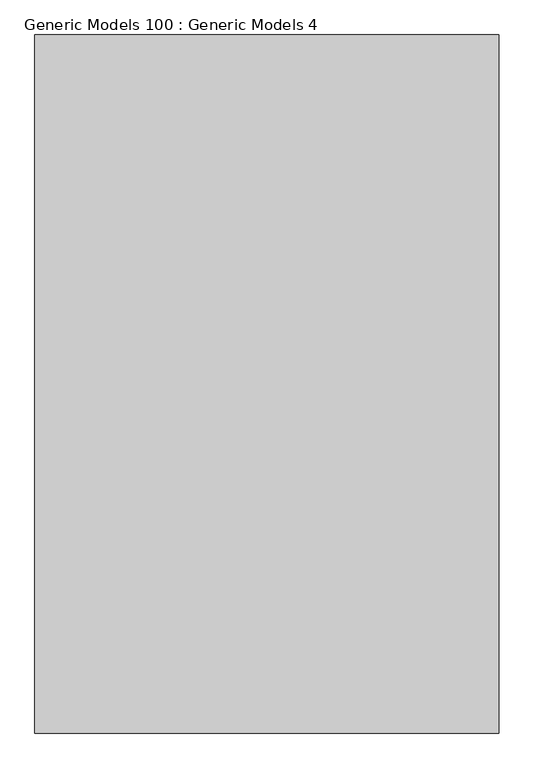
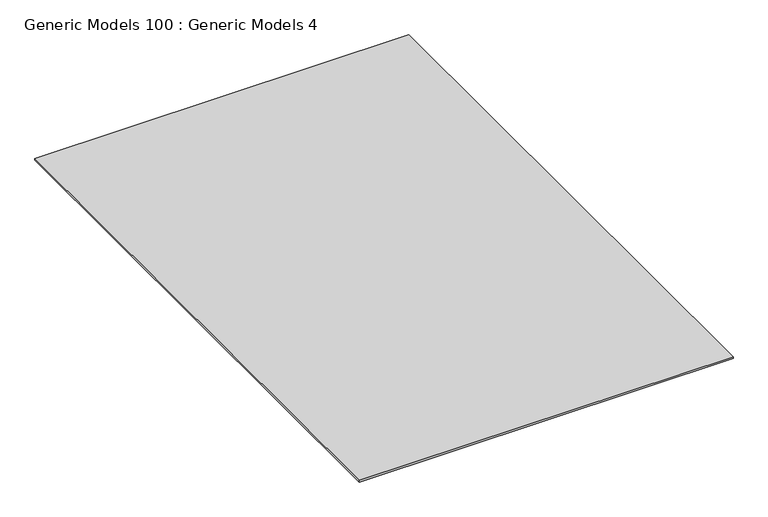
"""IFC4 building model written with IfcOpenShell, lengths in millimetres: proxy geometry, Generic Models 100 : Generic Models 4."""

from ifc_helpers import new_model, si_unit, frame, origin, place, context, project, spatial, polyline, outline, extrude, source, transform, mapped, element, save


def generic_models_100_generic_models_4_666ded77(model_context):
    return source(origin(), model_context, "Body", "SweptSolid", [
        extrude(outline(polyline([(-2201.0836295, -6864.9230338), (-6458.1236296, -6864.9230338), (-6458.1236296, -464.1230338), (-2201.0836295, -464.1230338), (-2201.0836295, -6864.9230338)])), frame((0.0, 0.0, 126783.846), z_axis=(0.0, 0.0, 1.0), x_axis=(1.0, 0.0, 0.0)), (0.0, 0.0, 1.0), 19.05),
    ])


if __name__ == "__main__":
    model = new_model("IFC4")
    model_context = context("Model", 3, world=origin())
    ifc_project = project(units=[si_unit("LENGTHUNIT", "METRE", prefix="MILLI")], contexts=[model_context])
    site = spatial("IfcSite", under=ifc_project)
    building = spatial("IfcBuilding", under=site)
    placement = place(None, origin())
    generic_models_100_generic_models_4_shape = generic_models_100_generic_models_4_666ded77(model_context)
    element("IfcBuildingElementProxy", 1, Name="Generic Models 100 : Generic Models 4", ObjectType="Generic Models 100 : Generic Models 4", at=placement, inside=building, context=model_context, shape_type="MappedRepresentation", body=[
        mapped(generic_models_100_generic_models_4_shape, transform((0.0, 0.0, 0.0), x_axis=(1.0, 0.0, 0.0), y_axis=(0.0, 1.0, 0.0), z_axis=(0.0, 0.0, 1.0))),
    ])
    save(model, "model.ifc")

# Revit data of these elements
# Element 1 (IfcBuildingElementProxy, "Generic Models 100 : Generic Models 4")
#   Materials on its faces: "_WOOD FLOORING (SPEC T.B.D.)"
# Materials
#   "_WOOD FLOORING (SPEC T.B.D.)": class "Generic", colour RGB 177 130 114, transparency 0, Cost = 0
